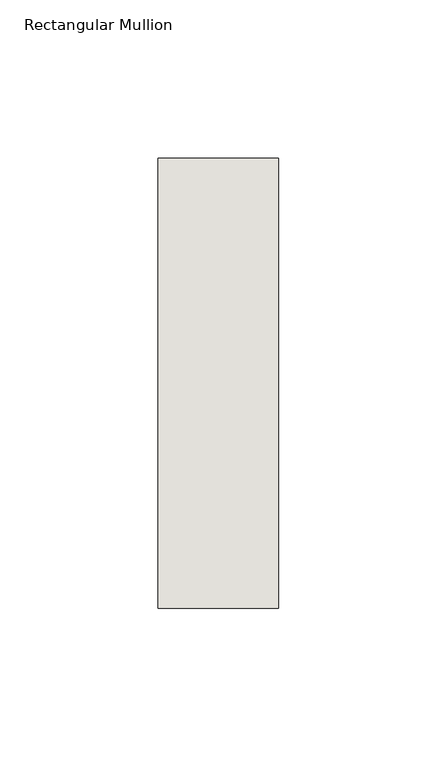
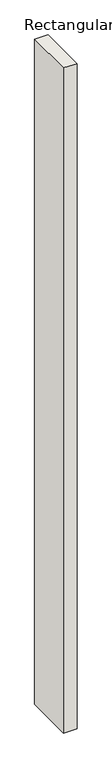
"""IFC4 building model written with IfcOpenShell, lengths in millimetres: wall geometry, Rectangular Mullion : NLRS_21_CWM_hsb-regel 38x142_gen_rsf."""

from ifc_helpers import new_model, si_unit, frame, origin, place, context, project, spatial, polyline, outline, extrude, source, transform, mapped, element, save


def rectangular_mullion_69aae0b8(model_context):
    return source(origin(), model_context, "Body", "SweptSolid", [
        extrude(outline(polyline([(0.0, -71.0), (-38.0, -71.0), (-38.0, 71.0), (0.0, 71.0), (0.0, -71.0)])), frame((0.0, 0.0, -2000.0), z_axis=(0.0, 0.0, 1.0), x_axis=(1.0, 0.0, 0.0)), (0.0, 0.0, 1.0), 2000.0),
    ])


if __name__ == "__main__":
    model = new_model("IFC4")
    model_context = context("Model", 3, world=origin())
    ifc_project = project(units=[si_unit("LENGTHUNIT", "METRE", prefix="MILLI")], contexts=[model_context])
    site = spatial("IfcSite", under=ifc_project)
    building = spatial("IfcBuilding", under=site)
    placement = place(None, origin())
    rectangular_mullion_shape = rectangular_mullion_69aae0b8(model_context)
    element("IfcWall", 1, ObjectType="Rectangular Mullion : NLRS_21_CWM_hsb-regel 38x142_gen_rsf", at=placement, inside=building, context=model_context, shape_type="MappedRepresentation", body=[
        mapped(rectangular_mullion_shape, transform((0.0, 0.0, 0.0), x_axis=(1.0, 0.0, 0.0), y_axis=(0.0, 1.0, 0.0), z_axis=(0.0, 0.0, 1.0))),
    ])
    save(model, "model.ifc")

# Revit data of these elements
# Type "Rectangular Mullion : NLRS_21_CWM_hsb-regel 38x142_gen_rsf"
#   Type IfcGUID = "07M7mRoiH1CR8m_RSKIwpF"
#   Assembly Code = "21.10"
#   IfcExportAs = "IfcWall"
#   built-in parameter 1007322 = 0.465879 (stored number, unit not read)
#   built-in parameter 1007321 = 0.062336 (stored number, unit not read)
#   built-in parameter 1007320 = 0.062336 (stored number, unit not read)
# Element 1 (IfcWall, "Rectangular Mullion : NLRS_21_CWM_hsb-regel 38x142_gen_rsf")
#   Materials on its faces: "NLRS_i2_hout naaldhout vuren_gen_rsf"
# Materials
#   "NLRS_i2_hout naaldhout vuren_gen_rsf": class "I - Hout", colour RGB 234 199 147, transparency 0, Keynote = "i2", Manufacturer = "Revit Standards Foundation", URL = "www.revitstandards.org", Description = "hout vuren", Cost = 0
